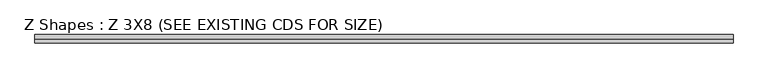
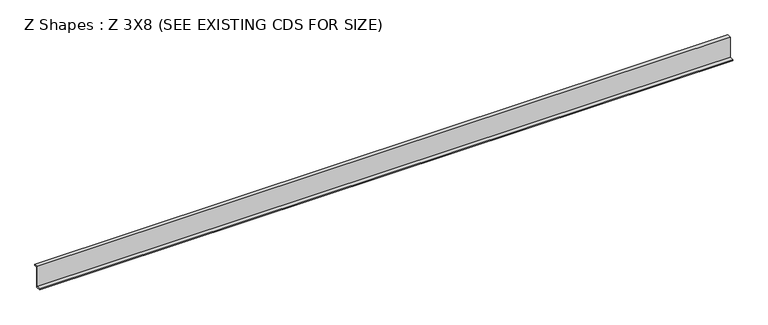
"""IFC4 building model written with IfcOpenShell, lengths in millimetres: beam geometry, Z Shapes : Z 3X8 (SEE EXISTING CDS FOR SIZE)."""

from ifc_helpers import new_model, si_unit, frame, origin, place, context, project, spatial, polyline, outline, extrude, source, transform, mapped, element, save


def z_shapes_z_3x8_see_existing_cds_for_size_0715a825(model_context):
    return source(origin(), model_context, "Body", "SweptSolid", [
        extrude(outline(polyline([(57.2805719, 91.944825), (25.0225719, 91.944825), (25.0225719, -101.603175), (-18.9194281, -101.603175), (-18.9194281, -91.951175), (19.1805719, -91.951175), (19.1805719, 101.596825), (57.2805719, 101.596825), (57.2805719, 91.944825)])), frame((-3168.65, 0.0, 0.0), z_axis=(1.0, 0.0, 0.0), x_axis=(0.0, 1.0, 0.0)), (0.0, 0.0, 1.0), 6337.3),
    ])


if __name__ == "__main__":
    model = new_model("IFC4")
    model_context = context("Model", 3, world=origin())
    ifc_project = project(units=[si_unit("LENGTHUNIT", "METRE", prefix="MILLI")], contexts=[model_context])
    site = spatial("IfcSite", under=ifc_project)
    building = spatial("IfcBuilding", under=site)
    placement = place(None, origin())
    z_shapes_z_3x8_see_existing_cds_for_size_shape = z_shapes_z_3x8_see_existing_cds_for_size_0715a825(model_context)
    element("IfcBeam", 1, ObjectType="Z Shapes : Z 3X8 (SEE EXISTING CDS FOR SIZE)", at=placement, inside=building, context=model_context, shape_type="MappedRepresentation", body=[
        mapped(z_shapes_z_3x8_see_existing_cds_for_size_shape, transform((0.0, 0.0, 0.0), x_axis=(1.0, 0.0, 0.0), y_axis=(0.0, 1.0, 0.0), z_axis=(0.0, 0.0, 1.0))),
    ])
    save(model, "model.ifc")

# Revit data of these elements
# Type "Z Shapes : Z 3X8 (SEE EXISTING CDS FOR SIZE)"
#   Section Name Key = "W12x26"
#   Assembly Code = "B10"
#   Width = 76.2 mm
#   Web Thickness = 5.842 mm
#   Web Fillet = 7.62 mm
#   Warping Constant = 163001.3 cm⁶
#   Torsional Moment of Inertia = 12.4869 cm⁴
#   Section Area = 7.65 in²
#   Plastic Modulus weak axis = 0.00472801 (stored number, unit not read)
#   Plastic Modulus strong axis = 0.0215278 (stored number, unit not read)
#   Perimeter = 15.0571 m²/m
#   Nominal Weight = 379.441 N/m
#   Moment of Inertia weak axis = 720.08 cm⁴
#   Moment of Inertia strong axis = 8491.12 cm⁴
#   Height = 203.2 mm
#   Flange Thickness = 9.652 mm
#   Elastic Modulus weak axis = 0.00309028 (stored number, unit not read)
#   Elastic Modulus strong axis = 0.0193287 (stored number, unit not read)
#   Centroid Vertical = 101.6 mm
#   Centroid Horizontal = 38.1 mm
#   Length [instance default] = 5' - 0"
#   Structural Material [instance default] = Steel ASTM A992
#   Principal Axes Angle = 0
# Element 1 (IfcBeam, "Z Shapes : Z 3X8 (SEE EXISTING CDS FOR SIZE)")
#   Structural Material = PAINTED STEEL
#   Materials on its faces: "PAINTED STEEL"
# Materials
#   "Steel ASTM A992": class "Metal", colour RGB 189 187 185, transparency 0, Description = "Structural steel 50ksi", Cost = 0
#   "PAINTED STEEL": class "Generic", colour RGB 120 120 120, transparency 0, Cost = 0
